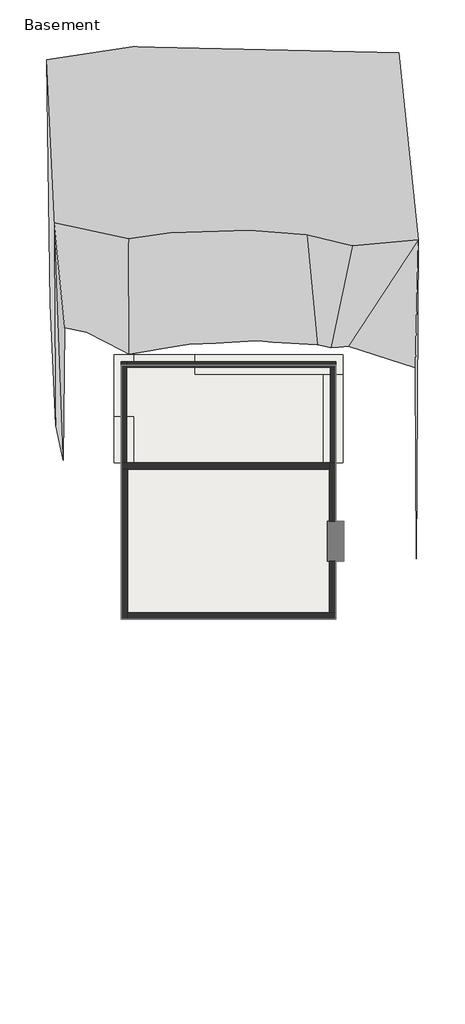
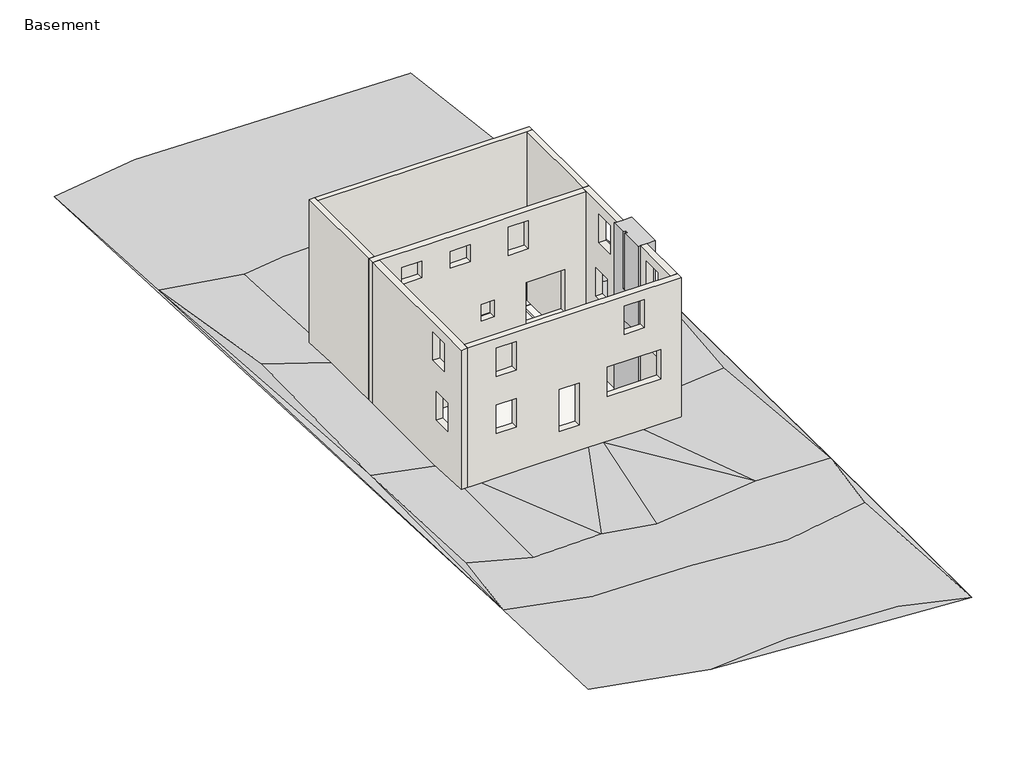
# One storey: 8 walls, 4 proxies, 3 footings, 2 slabs.
"""IFC4 building model written with IfcOpenShell, lengths in millimetres."""

import ifcopenshell
import ifcopenshell.guid

model = None  # the IFC model being written
_history = None  # IfcOwnerHistory: only IFC2X3 demands one
_inside = {}  # id of a spatial element -> (the spatial element, [elements in it])
_under = {}  # id of a project, library or spatial element -> (it, [spatial elements below it])
_declared = {}  # id of a project -> (the project, [libraries it declares])
_typed = {}  # id of a type object -> (the type object, [elements of that type])
_made_of = {}  # id of a material, layer set ... -> (it, [elements and type objects made of it])


def new_model(schema):
    """Start an empty IFC model of exactly this schema.

    Asked for "IFC4X3", IfcOpenShell would pick the latest addendum, in which some entities
    have other attributes; the version numbers below select the first issue.
    IFC2X3 requires an IfcOwnerHistory on every rooted entity: one is made here for all.
    """
    global model, _history
    if schema == "IFC4X3":
        model = ifcopenshell.file(schema_version=(4, 3, 0, 0))
    else:
        model = ifcopenshell.file(schema=schema)
    _inside.clear()
    _under.clear()
    _declared.clear()
    _typed.clear()
    _made_of.clear()
    _history = None
    if model.schema == "IFC2X3":
        org = make("IfcOrganization", Name="unknown")
        user = make(
            "IfcPersonAndOrganization",
            ThePerson=make("IfcPerson", FamilyName="unknown"),
            TheOrganization=org,
        )
        app = make(
            "IfcApplication",
            ApplicationDeveloper=org,
            Version="unknown",
            ApplicationFullName="unknown",
            ApplicationIdentifier="unknown",
        )
        _history = make(
            "IfcOwnerHistory",
            OwningUser=user,
            OwningApplication=app,
            ChangeAction="ADDED",
            CreationDate=0,
        )
    return model


def make(cls, **values):
    """One entity of the class cls with the attributes given. An attribute that is None is left unset."""
    return model.create_entity(
        cls, **{name: value for name, value in values.items() if value is not None}
    )


def rooted(cls, **values):
    """An entity with a GlobalId (a new one), such as an element, a storey or a relation."""
    return make(cls, GlobalId=ifcopenshell.guid.new(), OwnerHistory=_history, **values)


def si_unit(unit_type, name, prefix=None):
    """IfcSIUnit, for example si_unit("LENGTHUNIT", "METRE", prefix="MILLI")."""
    return make("IfcSIUnit", UnitType=unit_type, Prefix=prefix, Name=name)


def assignment(units):
    """IfcUnitAssignment: the units of a project."""
    return None if units is None else make("IfcUnitAssignment", Units=units)


def point(xyz):
    """IfcCartesianPoint."""
    return None if xyz is None else make("IfcCartesianPoint", Coordinates=xyz)


def direction(xyz):
    """IfcDirection."""
    return None if xyz is None else make("IfcDirection", DirectionRatios=xyz)


def frame(location, z_axis=None, x_axis=None):
    """IfcAxis2Placement3D, a coordinate frame: its origin and axes. An axis left out is left unset."""
    return make(
        "IfcAxis2Placement3D",
        Location=point(location),
        Axis=direction(z_axis),
        RefDirection=direction(x_axis),
    )


def origin():
    """The frame at (0, 0, 0) with its axes left unset."""
    return frame((0.0, 0.0, 0.0))


def place(relative_to, where):
    """IfcLocalPlacement: puts the frame where relative to a parent placement (None: the world)."""
    return make(
        "IfcLocalPlacement", PlacementRelTo=relative_to, RelativePlacement=where
    )


def context(
    kind, dimensions, precision=None, world=None, true_north=None, identifier=None
):
    """IfcGeometricRepresentationContext, for example the 3D "Model" context."""
    return make(
        "IfcGeometricRepresentationContext",
        ContextIdentifier=identifier,
        ContextType=kind,
        CoordinateSpaceDimension=dimensions,
        Precision=precision,
        WorldCoordinateSystem=world,
        TrueNorth=true_north,
    )


def project(units=None, contexts=None):
    """IfcProject with its units and contexts."""
    return rooted(
        "IfcProject",
        Name="project",
        RepresentationContexts=contexts,
        UnitsInContext=assignment(units),
    )


def spatial(cls, under=None, at=None, **own):
    """A site, building, storey or space (cls), placed at a placement, below another one or the project."""
    s = rooted(cls, ObjectPlacement=at, **own)
    if under is not None:
        _under.setdefault(under.id(), (under, []))[1].append(s)
    return s


def polyline(points):
    """IfcPolyline through the points."""
    return make("IfcPolyline", Points=[point(p) for p in points])


def point_list(points):
    """IfcCartesianPointList2D or 3D."""
    cls = (
        "IfcCartesianPointList2D" if len(points[0]) == 2 else "IfcCartesianPointList3D"
    )
    return make(cls, CoordList=points)


def outline(outer, holes=None, kind="AREA"):
    """IfcArbitraryClosedProfileDef: a profile drawn as a closed curve; with holes, ...WithVoids."""
    if holes is None:
        return make("IfcArbitraryClosedProfileDef", ProfileType=kind, OuterCurve=outer)
    return make(
        "IfcArbitraryProfileDefWithVoids",
        ProfileType=kind,
        OuterCurve=outer,
        InnerCurves=holes,
    )


def extrude(swept, where, along, depth):
    """IfcExtrudedAreaSolid: the profile swept, set in the frame where, extruded along a direction by depth."""
    return make(
        "IfcExtrudedAreaSolid",
        SweptArea=swept,
        Position=where,
        ExtrudedDirection=direction(along),
        Depth=depth,
    )


def faces_of(points, faces, orient=None, outer=None):
    """IfcFace entities. A face is a list of loops; a loop is a list of indices into points, from 0.

    orient and outer hold one flag for each loop. By default every Orientation is true, the
    first loop of a face is its IfcFaceOuterBound and the others are IfcFaceBound.
    """
    made = []
    for i, loops in enumerate(faces):
        bounds = []
        for j, loop in enumerate(loops):
            is_outer = j == 0 if outer is None else outer[i][j]
            bounds.append(
                make(
                    "IfcFaceOuterBound" if is_outer else "IfcFaceBound",
                    Bound=make("IfcPolyLoop", Polygon=[points[k] for k in loop]),
                    Orientation=True if orient is None else orient[i][j],
                )
            )
        made.append(make("IfcFace", Bounds=bounds))
    return made


def faceted_brep(points, faces, orient=None, outer=None, voids=None):
    """IfcFacetedBrep: a solid bounded by flat faces; with voids (closed shells), ...WithVoids."""
    shared = [point(p) for p in points]
    hull = make("IfcClosedShell", CfsFaces=faces_of(shared, faces, orient, outer))
    if voids is None:
        return make("IfcFacetedBrep", Outer=hull)
    return make(
        "IfcFacetedBrepWithVoids",
        Outer=hull,
        Voids=[
            make(cls, CfsFaces=faces_of(shared, fs, o, b)) for cls, fs, o, b in voids
        ],
    )


def triangles(points, corners, closed=None, point_numbers=None):
    """IfcTriangulatedFaceSet: each triangle names its three corners, points numbered from 1."""
    return make(
        "IfcTriangulatedFaceSet",
        Coordinates=point_list(points),
        Closed=closed,
        CoordIndex=corners,
        PnIndex=point_numbers,
    )


def shape(context_of_items, identifier, shape_type, items):
    """IfcShapeRepresentation: the items that make up one representation, for example the "Body"."""
    return make(
        "IfcShapeRepresentation",
        ContextOfItems=context_of_items,
        RepresentationIdentifier=identifier,
        RepresentationType=shape_type,
        Items=items,
    )


def source(mapping_origin, context_of_items, identifier, shape_type, items):
    """IfcRepresentationMap: a shape defined once, which mapped items show again and again."""
    return make(
        "IfcRepresentationMap",
        MappingOrigin=mapping_origin,
        MappedRepresentation=shape(context_of_items, identifier, shape_type, items),
    )


def transform(
    local_origin,
    x_axis=None,
    y_axis=None,
    z_axis=None,
    scale=None,
    scale2=None,
    scale3=None,
    uniform=True,
):
    """IfcCartesianTransformationOperator3D, or its non-uniform kind. x_axis, y_axis, z_axis: its Axis1, 2, 3."""
    if uniform:
        return make(
            "IfcCartesianTransformationOperator3D",
            Axis1=direction(x_axis),
            Axis2=direction(y_axis),
            LocalOrigin=point(local_origin),
            Scale=scale,
            Axis3=direction(z_axis),
        )
    return make(
        "IfcCartesianTransformationOperator3DnonUniform",
        Axis1=direction(x_axis),
        Axis2=direction(y_axis),
        LocalOrigin=point(local_origin),
        Scale=scale,
        Axis3=direction(z_axis),
        Scale2=scale2,
        Scale3=scale3,
    )


def mapped(mapping_source, mapping_target):
    """IfcMappedItem: shows the shape of a source again, moved by a transform."""
    return make(
        "IfcMappedItem", MappingSource=mapping_source, MappingTarget=mapping_target
    )


def made_of(thing, what):
    """Note that an element or type object is made of a material, layer set ...; save() writes the relation."""
    if what is not None:
        _made_of.setdefault(what.id(), (what, []))[1].append(thing)
    return thing


def element(
    cls,
    number,
    at=None,
    inside=None,
    cuts=None,
    type_object=None,
    material=None,
    context=None,
    identifier="Body",
    shape_type=None,
    held_by="IfcProductDefinitionShape",
    body=None,
    shapes=None,
    **own,
):
    """One element of the class cls, such as IfcWall. Its Tag is "e" and its number.

    at: its placement. inside: the storey or other place that contains it. cuts: it is an
    opening in that element (IfcRelVoidsElement). A single representation is given by context,
    identifier, shape_type and body (its items); several are given by shapes. held_by: the class
    of the entity that holds the representations. save() writes the other relations.
    """
    e = rooted(cls, Tag="e%d" % number, ObjectPlacement=at, **own)
    if body is not None:
        shapes = [shape(context, identifier, shape_type, body)]
    if shapes is not None:
        e.Representation = make(held_by, Representations=shapes)
    if inside is not None:
        _inside.setdefault(inside.id(), (inside, []))[1].append(e)
    if cuts is not None:
        rooted(
            "IfcRelVoidsElement", RelatingBuildingElement=cuts, RelatedOpeningElement=e
        )
    if type_object is not None:
        _typed.setdefault(type_object.id(), (type_object, []))[1].append(e)
    return made_of(e, material)


def aggregate(whole, parts):
    """IfcRelAggregates: a whole, such as a stair, and the parts it consists of."""
    return rooted("IfcRelAggregates", RelatingObject=whole, RelatedObjects=parts)


def save(model, path):
    """Write the relations noted so far, then the file.

    IfcRelAggregates (storeys below a building ...), IfcRelContainedInSpatialStructure (elements
    in a storey), IfcRelDefinesByType, IfcRelAssociatesMaterial and IfcRelDeclares: one each for
    every whole, place, type object, material and project.
    """
    for whole, parts in _under.values():
        aggregate(whole, parts)
    for where, things in _inside.values():
        rooted(
            "IfcRelContainedInSpatialStructure",
            RelatedElements=things,
            RelatingStructure=where,
        )
    for kind, things in _typed.values():
        rooted("IfcRelDefinesByType", RelatedObjects=things, RelatingType=kind)
    for what, things in _made_of.values():
        rooted("IfcRelAssociatesMaterial", RelatedObjects=things, RelatingMaterial=what)
    for by, libraries in _declared.values():
        rooted("IfcRelDeclares", RelatingContext=by, RelatedDefinitions=libraries)
    model.write(path)


def existing_fireplace_existing_fireplace_063a625f(model_context):
    return source(origin(), model_context, "Body", "Brep", [
        faceted_brep([(4450.2196932, 434.2888758, 5486.4), (4069.2196932, 434.2888758, 5486.4), (3764.4196932, 434.2888758, 5486.4), (3662.8196932, 434.2888758, 5486.4), (3662.8196932, -276.9111242, 5486.4), (3767.2567114, -276.9111242, 5486.4), (3767.2567114, -403.9111242, 5486.4), (3662.8196932, -403.9111242, 5486.4), (3662.8196932, -1445.3111242, 5486.4), (3764.4196932, -1445.3111242, 5486.4), (4069.2196932, -1445.3111242, 5486.4), (4450.2196932, -1445.3111242, 5486.4), (4450.2196932, 434.2888758, -2667.0), (4450.2196932, -1445.3111242, -2667.0), (4069.2196932, -1445.3111242, -2667.0), (3764.4196932, -1445.3111242, -2667.0), (3662.8196932, -1445.3111242, -2667.0), (3662.8196932, 434.2888758, -2667.0), (3764.4196932, 434.2888758, -2667.0), (4069.2196932, 434.2888758, -2667.0), (3662.8196932, -403.9111242, 2743.2), (3662.8196932, -276.9111242, 2743.2), (3662.8196932, 154.8888758, 0.0), (3662.8196932, 154.8888758, 1219.2), (3662.8196932, -1165.9111242, 1219.2), (3662.8196932, -1165.9111242, 0.0), (4145.4196932, -20.7631592, 1219.2), (4145.4196932, -990.2590891, 1219.2), (4145.4196932, -990.2590891, 0.0), (4145.4196932, -20.7631592, 0.0), (3767.2567114, -403.9111242, 2743.2), (3767.2567114, -276.9111242, 2743.2)], [[[0, 1, 2, 3, 4, 5, 6, 7, 8, 9, 10, 11]], [[12, 13, 14, 15, 16, 17, 18, 19]], [[3, 2, 1, 0, 12, 19, 18, 17]], [[3, 17, 16, 8, 7, 20, 21, 4], [22, 23, 24, 25]], [[11, 10, 9, 8, 16, 15, 14, 13]], [[0, 11, 13, 12]], [[24, 23, 26, 27]], [[25, 24, 27, 28]], [[27, 26, 29, 28]], [[23, 22, 29, 26]], [[22, 25, 28, 29]], [[6, 30, 20, 7]], [[31, 5, 4, 21]], [[30, 31, 21, 20]], [[30, 6, 5, 31]]]),
    ])


model = new_model("IFC4")

# Units and contexts
model_context = context("Model", 3, world=origin())
ifc_project = project(units=[si_unit("LENGTHUNIT", "METRE", prefix="MILLI")], contexts=[model_context])

# Site, building, storey
site = spatial("IfcSite", under=ifc_project)
building = spatial("IfcBuilding", under=site)
storey = spatial("IfcBuildingStorey", under=building, Name="Basement", Elevation=-2667.0)

# Proxies
placement = place(None, origin())
element("IfcBuildingElementProxy", 1, Name="Building Element Proxy", at=placement, inside=storey, context=model_context, shape_type="Tessellation", body=[
    triangles([(-9474.14729, 22003.2871765, -1727.1999516), (-8916.1412338, -12566.1132111, -939.7999758), (-8632.7724838, -18803.3999359, -1092.1999758), (-3754.3850807, -20036.8885986, -1092.1999758), (7677.2023224, -20906.8378235, -1092.1999758), (7936.7585724, 13587.9496765, -1752.6), (7012.0400162, 22339.8364014, -1727.1999516), (-5437.1349838, 22620.8239014, -1727.1999516), (4069.2196426, 434.2888621, -1346.1999516), (4450.2196426, 434.2888621, -1346.1999516), (4450.2196426, -349.5066825, -1346.1999516), (4450.2196426, -1445.3110531, -1346.1999516), (4069.2196426, -1445.3110531, -1346.1999516), (4069.2196426, -2313.9084709, -1346.1999516), (4069.2196426, -4163.1110046, -1246.6980309), (3428.5651428, -4163.1110046, -1250.4688763), (2349.5500454, -4163.1110046, -1257.7835461), (502.5996998, -4163.1110046, -1235.211668), (-175.7374563, -4163.1110046, -1228.3558365), (-2922.786422, -4163.1110046, -1226.4072636), (-5055.1879486, -4163.1110046, -1242.8984081), (-5852.784613, -4163.1110046, -1243.6517052), (-5989.1803574, -4163.1110046, -1240.8027512), (-5989.1803574, -2711.9263275, -1314.8636375), (-5989.1803574, -2124.4043404, -1346.1999516), (-5989.1803574, 3152.0889954, -1346.1999516), (-5989.1803574, 4989.0600082, -1346.1999516), (-5989.1803574, 6156.3282944, -1346.1999516), (-5989.1803574, 7724.0889954, -1429.2445919), (-5611.7969971, 7724.0889954, -1439.6358181), (-2815.8938187, 7724.0889954, -1415.0254017), (-2474.4123367, 7724.0889954, -1412.4145145), (-1876.9665367, 7724.0889954, -1411.4359406), (391.3462071, 7724.0889954, -1403.6252254), (781.867392, 7724.0889954, -1405.4288944), (3306.7437996, 7724.0889954, -1413.4377079), (3676.8014442, 7724.0889954, -1418.4369667), (4069.2196426, 7724.0889954, -1416.2554138), (4069.2196426, 7529.9159637, -1404.4058464), (4069.2196426, 6299.0253983, -1346.1999516), (4069.2196426, 3152.0889954, -1346.1999516), (-9109.81604, 14372.1750641, -1752.6), (-8549.4287338, -9013.2876297, -939.7999758), (-8523.2349838, -1401.2252266, -1346.1999516), (-8408.9349838, 7414.1625641, -1346.1999516), (-6082.4537338, -10022.9382111, -939.7999758), (-5633.19104, 13643.5125641, -1752.6), (-5382.3662338, -13518.6132111, -939.7999758), (-3671.0413307, 13924.5000641, -1752.6), (-2942.3788307, -9965.7882111, -939.7999758), (-1568.3975807, 21947.7254517, -1727.1999516), (-840.5287823, -13629.7378235, -939.7999758), (-699.241258, -10470.6132111, -939.7999758), (-109.4850414, -19700.3370483, -1092.1999758), (29.4212079, 14035.6246765, -1752.6), (2721.8210724, 13811.7871765, -1752.6), (2805.1648224, 21892.1614014, -1727.1999516), (3252.0462662, -14021.8499359, -939.7999758), (4179.1460724, -9854.6624359, -939.7999758), (4845.1025162, -19962.2745483, -1092.1999758), (4852.2462662, 13306.9621765, -1752.6), (7177.93396, -13294.7757111, -939.7999758), (7289.85271, -1961.6126781, -1346.1999516), (7543.0587662, -9965.7882111, -939.7999758), (7740.7025162, 5059.8998703, -1346.1999516)], [[46, 2, 48], [43, 46, 23], [46, 43, 2], [2, 3, 48], [2, 43, 44], [43, 23, 44], [23, 46, 22], [44, 23, 24], [46, 21, 22], [44, 24, 25], [48, 4, 52], [4, 48, 3], [48, 52, 50], [19, 53, 18], [4, 54, 52], [50, 52, 53], [21, 50, 20], [21, 46, 50], [19, 20, 50], [50, 53, 19], [53, 52, 58], [50, 46, 48], [45, 27, 28], [26, 27, 45], [44, 26, 45], [25, 26, 44], [8, 1, 42], [1, 2, 42], [42, 45, 47], [29, 45, 28], [42, 44, 45], [29, 47, 45], [42, 2, 44], [47, 30, 31], [31, 32, 49], [33, 49, 32], [47, 8, 42], [8, 47, 49], [49, 51, 8], [55, 51, 49], [47, 31, 49], [8, 51, 57], [55, 49, 33], [30, 47, 29], [58, 59, 53], [58, 54, 60], [59, 15, 16], [59, 18, 53], [16, 17, 59], [59, 17, 18], [12, 13, 14], [14, 15, 63], [58, 62, 59], [62, 60, 5], [64, 5, 65], [5, 64, 62], [60, 54, 5], [59, 62, 64], [59, 64, 15], [12, 63, 11], [12, 14, 63], [64, 63, 15], [11, 63, 10], [64, 65, 63], [62, 58, 60], [54, 4, 5], [55, 34, 35], [56, 35, 36], [55, 56, 57], [55, 35, 56], [37, 61, 36], [56, 61, 57], [56, 36, 61], [55, 57, 51], [55, 33, 34], [40, 41, 65], [10, 65, 41], [65, 10, 63], [41, 9, 10], [40, 65, 39], [39, 65, 38], [61, 6, 7], [6, 61, 38], [61, 7, 57], [65, 6, 38], [38, 61, 37], [65, 5, 6], [57, 7, 8], [52, 54, 58]], closed=False),
])
element("IfcBuildingElementProxy", 2, Name="Building Element Proxy", at=placement, inside=storey, context=model_context, shape_type="Tessellation", body=[
    triangles([(4069.2196426, 3152.0889954, -3073.5594864), (4069.2196426, 3152.0889954, -1346.1999516), (4069.2196426, 434.2888621, -3073.5594864), (4069.2196426, 434.2888621, -1346.1999516), (4450.2196426, 434.2888621, -3073.5594864), (4450.2196426, 434.2888621, -1346.1999516), (4450.2196426, -349.5066825, -3073.5594864), (4450.2196426, -349.5066825, -1346.1999516), (4450.2196426, -1445.3110531, -3073.5594864), (4450.2196426, -1445.3110531, -1346.1999516), (4069.2196426, -1445.3110531, -3073.5594864), (4069.2196426, -1445.3110531, -1346.1999516), (4069.2196426, -2313.9084709, -3073.5594864), (4069.2196426, -2313.9084709, -1346.1999516), (4069.2196426, -4163.1110046, -3073.5594864), (4069.2196426, -4163.1110046, -1246.6980309), (3428.5651428, -4163.1110046, -3073.5594864), (3428.5651428, -4163.1110046, -1250.4688763), (2349.5500454, -4163.1110046, -3073.5594864), (2349.5500454, -4163.1110046, -1257.7835461), (502.5996998, -4163.1110046, -3073.5594864), (502.5996998, -4163.1110046, -1235.211668), (-175.7374563, -4163.1110046, -3073.5594864), (-175.7374563, -4163.1110046, -1228.3558365), (-2922.786422, -4163.1110046, -3073.5594864), (-2922.786422, -4163.1110046, -1226.4072636), (-5055.1879486, -4163.1110046, -3073.5594864), (-5055.1879486, -4163.1110046, -1242.8984081), (-5852.784613, -4163.1110046, -3073.5594864), (-5852.784613, -4163.1110046, -1243.6517052), (-5989.1803574, -4163.1110046, -3073.5594864), (-5989.1803574, -4163.1110046, -1240.8027512), (-5989.1803574, -2711.9263275, -3073.5594864), (-5989.1803574, -2711.9263275, -1314.8636375), (-5989.1803574, -2124.4043404, -3073.5594864), (-5989.1803574, -2124.4043404, -1346.1999516), (-5989.1803574, 3152.0889954, -3073.5594864), (-5989.1803574, 3152.0889954, -1346.1999516)], [[1, 4, 2], [1, 3, 4], [3, 6, 4], [3, 5, 6], [5, 8, 6], [5, 7, 8], [7, 10, 8], [7, 9, 10], [9, 12, 10], [9, 11, 12], [11, 14, 12], [11, 13, 14], [13, 16, 14], [13, 15, 16], [15, 18, 16], [15, 17, 18], [17, 20, 18], [17, 19, 20], [19, 22, 20], [19, 21, 22], [21, 24, 22], [21, 23, 24], [23, 26, 24], [23, 25, 26], [25, 28, 26], [25, 27, 28], [27, 30, 28], [27, 29, 30], [29, 32, 30], [29, 31, 32], [31, 34, 32], [31, 33, 34], [33, 36, 34], [33, 35, 36], [35, 38, 36], [35, 37, 38]], closed=False),
    triangles([(4069.2196426, 434.2888621, -3073.5594864), (4069.2196426, 3152.0889954, -3073.5594864), (-5989.1803574, 3152.0889954, -3073.5594864), (-5989.1803574, -4163.1110046, -3073.5594864), (4069.2196426, -4163.1110046, -3073.5594864), (4069.2196426, -1445.3110531, -3073.5594864), (4450.2196426, -1445.3110531, -3073.5594864), (4450.2196426, 434.2888621, -3073.5594864)], [[4, 6, 3], [6, 4, 5], [3, 1, 2], [1, 3, 6], [6, 7, 1], [8, 1, 7]], closed=False),
])
element("IfcBuildingElementProxy", 3, Name="Building Element Proxy", at=placement, inside=storey, context=model_context, shape_type="Tessellation", body=[
    triangles([(-5989.1803574, 3152.0889954, -3073.5594864), (-5989.1803574, 3152.0889954, -1346.1999516), (-5989.1803574, 4989.0600082, -3073.5594864), (-5989.1803574, 4989.0600082, -1346.1999516), (-5989.1803574, 6156.3282944, -3073.5594864), (-5989.1803574, 6156.3282944, -1346.1999516), (-5989.1803574, 7724.0889954, -3073.5594864), (-5989.1803574, 7724.0889954, -1429.2445919), (-5611.7969971, 7724.0889954, -3073.5594864), (-5611.7969971, 7724.0889954, -1439.6358181), (-2815.8938187, 7724.0889954, -3073.5594864), (-2815.8938187, 7724.0889954, -1415.0254017), (-2474.4123367, 7724.0889954, -3073.5594864), (-2474.4123367, 7724.0889954, -1412.4145145), (-1876.9665367, 7724.0889954, -3073.5594864), (-1876.9665367, 7724.0889954, -1411.4359406), (391.3462071, 7724.0889954, -3073.5594864), (391.3462071, 7724.0889954, -1403.6252254), (781.867392, 7724.0889954, -3073.5594864), (781.867392, 7724.0889954, -1405.4288944), (3306.7437996, 7724.0889954, -3073.5594864), (3306.7437996, 7724.0889954, -1413.4377079), (3676.8014442, 7724.0889954, -3073.5594864), (3676.8014442, 7724.0889954, -1418.4369667), (4069.2196426, 7724.0889954, -3073.5594864), (4069.2196426, 7724.0889954, -1416.2554138), (4069.2196426, 7529.9159637, -3073.5594864), (4069.2196426, 7529.9159637, -1404.4058464), (4069.2196426, 6299.0253983, -3073.5594864), (4069.2196426, 6299.0253983, -1346.1999516), (4069.2196426, 3152.0889954, -3073.5594864), (4069.2196426, 3152.0889954, -1346.1999516)], [[1, 4, 2], [1, 3, 4], [3, 6, 4], [3, 5, 6], [5, 8, 6], [5, 7, 8], [7, 10, 8], [7, 9, 10], [9, 12, 10], [9, 11, 12], [11, 14, 12], [11, 13, 14], [13, 16, 14], [13, 15, 16], [15, 18, 16], [15, 17, 18], [17, 20, 18], [17, 19, 20], [19, 22, 20], [19, 21, 22], [21, 24, 22], [21, 23, 24], [23, 26, 24], [23, 25, 26], [25, 28, 26], [25, 27, 28], [27, 30, 28], [27, 29, 30], [29, 32, 30], [29, 31, 32]], closed=False),
    triangles([(-5989.1803574, 7724.0889954, -3073.5594864), (-5989.1803574, 3152.0889954, -3073.5594864), (4069.2196426, 3152.0889954, -3073.5594864), (4069.2196426, 7724.0889954, -3073.5594864)], [[1, 2, 4], [3, 4, 2]], closed=False),
])
existing_fireplace_existing_fireplace_shape = existing_fireplace_existing_fireplace_063a625f(model_context)
element("IfcBuildingElementProxy", 4, Name="Existing Fireplace : Existing Fireplace", ObjectType="Existing Fireplace : Existing Fireplace", at=placement, inside=storey, context=model_context, shape_type="MappedRepresentation", body=[
    mapped(existing_fireplace_existing_fireplace_shape, transform((0.0, 0.0, 0.0), x_axis=(1.0, 0.0, 0.0), y_axis=(0.0, 1.0, 0.0), z_axis=(0.0, 0.0, 1.0))),
])

# Footings
element("IfcFooting", 5, ObjectType="Bearing Footing - 36\" x 12\"", at=placement, inside=storey, context=model_context, shape_type="Brep", body=[
    faceted_brep([(-5404.9803068, 3152.0888758, -2667.0), (-6319.3803068, 3152.0888758, -2667.0), (-6319.3803068, 3152.0888758, -2971.8), (-5404.9803068, 3152.0888758, -2971.8), (-6319.3803068, 5311.0888758, -2667.0), (-5404.9803068, 5311.0888758, -2667.0), (-5404.9803068, 5311.0888758, -2971.8), (-6319.3803068, 5311.0888758, -2971.8)], [[[0, 1, 2, 3]], [[4, 5, 6, 7]], [[0, 5, 4, 1]], [[2, 1, 4, 7]], [[3, 2, 7, 6]], [[0, 3, 6, 5]]]),
    faceted_brep([(-5404.9803068, 5311.0888758, -3124.2), (-6319.3803068, 5311.0888758, -3124.2), (-6319.3803068, 5311.0888758, -3429.0), (-5404.9803068, 5311.0888758, -3429.0), (-5404.9803068, 7292.2888758, -3124.2), (-5404.9803068, 8206.6888758, -3124.2), (-6319.3803068, 8206.6888758, -3124.2), (-6319.3803068, 8206.6888758, -3429.0), (-5404.9803068, 8206.6888758, -3429.0), (-5404.9803068, 7292.2888758, -3429.0)], [[[0, 1, 2, 3]], [[0, 4, 5, 6, 1]], [[2, 1, 6, 7]], [[3, 2, 7, 8, 9]], [[0, 3, 9, 8, 5, 4]], [[6, 5, 8, 7]]]),
])
element("IfcFooting", 6, ObjectType="Bearing Footing - 36\" x 12\"", at=placement, inside=storey, context=model_context, shape_type="Brep", body=[
    faceted_brep([(-2509.3803068, 8206.6888758, -3429.0), (-2509.3803068, 8206.6888758, -3124.2), (-2509.3803068, 7292.2888758, -3124.2), (-2509.3803068, 7292.2888758, -3429.0), (-5404.9803068, 8206.6888758, -3124.2), (-5404.9803068, 7292.2888758, -3124.2), (-5404.9803068, 8206.6888758, -3429.0), (-5404.9803068, 7292.2888758, -3429.0)], [[[0, 1, 2, 3]], [[2, 1, 4, 5]], [[1, 0, 6, 4]], [[0, 3, 7, 6]], [[3, 2, 5, 7]], [[5, 4, 6, 7]]]),
    faceted_brep([(-2509.3803068, 8206.6888758, -2667.0), (-2509.3803068, 8206.6888758, -2971.8), (-2509.3803068, 7292.2888758, -2971.8), (-2509.3803068, 7292.2888758, -2667.0), (4399.4196932, 8206.6888758, -2667.0), (3485.0196932, 7292.2888758, -2667.0), (4399.4196932, 7292.2888758, -2667.0), (4399.4196932, 8206.6888758, -2971.8), (4399.4196932, 7292.2888758, -2971.8), (3485.0196932, 7292.2888758, -2971.8)], [[[0, 1, 2, 3]], [[4, 0, 3, 5, 6]], [[1, 0, 4, 7]], [[2, 1, 7, 8, 9]], [[3, 2, 9, 8, 6, 5]], [[4, 6, 8, 7]]]),
])
element("IfcFooting", 7, ObjectType="Bearing Footing - 36\" x 12\"", at=placement, inside=storey, context=model_context, shape_type="SweptSolid", body=[
    extrude(outline(polyline([(4399.4196932, 3152.0888758), (3485.0196932, 3152.0888758), (3485.0196932, 7292.2888758), (4399.4196932, 7292.2888758), (4399.4196932, 3152.0888758)])), frame((0.0, 0.0, -2971.8), z_axis=(0.0, 0.0, 1.0), x_axis=(1.0, 0.0, 0.0)), (0.0, 0.0, 1.0), 304.8),
])

# Slabs
element("IfcSlab", 8, ObjectType="Pad 1", at=placement, inside=storey, context=model_context, shape_type="SweptSolid", body=[
    extrude(outline(polyline([(4069.2196932, 434.2888758), (4450.2196932, 434.2888758), (4450.2196932, -1445.3111242), (4069.2196932, -1445.3111242), (4069.2196932, -4163.1111242), (-5989.1803068, -4163.1111242), (-5989.1803068, 3152.0888758), (4069.2196932, 3152.0888758), (4069.2196932, 434.2888758)])), frame((0.0, 0.0, -3073.4), z_axis=(0.0, 0.0, 1.0), x_axis=(1.0, 0.0, 0.0)), (0.0, 0.0, 1.0), 304.8),
])
element("IfcSlab", 9, ObjectType="Pad 1", at=placement, inside=storey, context=model_context, shape_type="SweptSolid", body=[
    extrude(outline(polyline([(-5989.1803068, 7724.0888758), (4069.2196932, 7724.0888758), (4069.2196932, 3152.0888758), (-5989.1803068, 3152.0888758), (-5989.1803068, 7724.0888758)])), frame((0.0, 0.0, -3073.4), z_axis=(0.0, 0.0, 1.0), x_axis=(1.0, 0.0, 0.0)), (0.0, 0.0, 1.0), 304.8),
])

# Walls
element("IfcWall", 10, ObjectType="Generic - 10\"", at=placement, inside=storey, context=model_context, shape_type="Brep", body=[
    faceted_brep([(-5735.1803068, 3152.0888758, -2667.0), (-5735.1803068, 5311.0888758, -2667.0), (-5735.1803068, 5311.0888758, -3124.2), (-5735.1803068, 7622.4888758, -3124.2), (-5735.1803068, 7876.4888758, -3124.2), (-5735.1803068, 7876.4888758, 5486.4), (-5735.1803068, 7622.4888758, 5486.4), (-5735.1803068, 3152.0888758, 5486.4), (-5989.1803068, 3152.0888758, -2667.0), (-5989.1803068, 3152.0888758, 5486.4), (-5989.1803068, 7876.4888758, 5486.4), (-5989.1803068, 7876.4888758, -3124.2), (-5989.1803068, 5311.0888758, -3124.2), (-5989.1803068, 5311.0888758, -2667.0)], [[[0, 1, 2, 3, 4, 5, 6, 7]], [[8, 9, 10, 11, 12, 13]], [[1, 0, 8, 13]], [[2, 1, 13, 12]], [[4, 3, 2, 12, 11]], [[7, 6, 5, 10, 9]], [[5, 4, 11, 10]], [[0, 7, 9, 8]]]),
])
element("IfcWall", 11, ObjectType="Generic - 10\"", at=placement, inside=storey, context=model_context, shape_type="Brep", body=[
    faceted_brep([(-5735.1803068, 7622.4888758, -3124.2), (-2509.3803068, 7622.4888758, -3124.2), (-2509.3803068, 7622.4888758, -2667.0), (3815.2196932, 7622.4888758, -2667.0), (4069.2196932, 7622.4888758, -2667.0), (4069.2196932, 7622.4888758, 5486.4), (3815.2196932, 7622.4888758, 5486.4), (-5735.1803068, 7622.4888758, 5486.4), (-5735.1803068, 7876.4888758, -3124.2), (-5735.1803068, 7876.4888758, 5486.4), (4069.2196932, 7876.4888758, 5486.4), (4069.2196932, 7876.4888758, -2667.0), (-2509.3803068, 7876.4888758, -2667.0), (-2509.3803068, 7876.4888758, -3124.2)], [[[0, 1, 2, 3, 4, 5, 6, 7]], [[8, 9, 10, 11, 12, 13]], [[1, 0, 8, 13]], [[2, 1, 13, 12]], [[4, 3, 2, 12, 11]], [[7, 6, 5, 10, 9]], [[5, 4, 11, 10]], [[0, 7, 9, 8]]]),
])
element("IfcWall", 12, ObjectType="Generic - 10\"", at=placement, inside=storey, context=model_context, shape_type="SweptSolid", body=[
    extrude(outline(polyline([(3815.2196932, 3152.0888758), (3815.2196932, 7622.4888758), (4069.2196932, 7622.4888758), (4069.2196932, 3152.0888758), (3815.2196932, 3152.0888758)])), frame((0.0, 0.0, -2667.0), z_axis=(0.0, 0.0, 1.0), x_axis=(1.0, 0.0, 0.0)), (0.0, 0.0, 1.0), 8153.4),
])
element("IfcWall", 13, ObjectType="Generic - 12\"", at=placement, inside=storey, context=model_context, shape_type="Brep", body=[
    faceted_brep([(-5989.1803068, 2847.2888758, -2667.0), (-5684.3803068, 2847.2888758, -2667.0), (3764.4196932, 2847.2888758, -2667.0), (3764.4196932, 2847.2888758, 5486.4), (56.0196932, 2847.2888758, 5486.4), (-70.9803068, 2847.2888758, 5486.4), (-680.5803068, 2847.2888758, 5486.4), (-807.5803068, 2847.2888758, 5486.4), (-3169.7803068, 2847.2888758, 5486.4), (-3296.7803068, 2847.2888758, 5486.4), (-5684.3803068, 2847.2888758, 5486.4), (-5989.1803068, 2847.2888758, 5486.4), (1021.2196932, 2847.2888758, 0.0), (1021.2196932, 2847.2888758, 2057.4), (2799.2196932, 2847.2888758, 2057.4), (2799.2196932, 2847.2888758, 0.0), (-4160.3803068, 2847.2888758, 0.0), (-5023.9803068, 2847.2888758, 0.0), (-5023.9803068, 2847.2888758, 2032.0), (-4160.3803068, 2847.2888758, 2032.0), (-1036.1803068, 2847.2888758, 914.4), (-1036.1803068, 2847.2888758, 1727.2), (-426.5803068, 2847.2888758, 1727.2), (-426.5803068, 2847.2888758, 914.4), (-3919.0803068, 2847.2888758, 914.4), (-3919.0803068, 2847.2888758, 1727.2), (-3004.6803068, 2847.2888758, 1727.2), (-3004.6803068, 2847.2888758, 914.4), (208.4196932, 2847.2888758, 3657.6), (208.4196932, 2847.2888758, 5029.2), (1122.8196932, 2847.2888758, 5029.2), (1122.8196932, 2847.2888758, 3657.6), (-2433.1803068, 2847.2888758, 3962.4), (-2433.1803068, 2847.2888758, 4775.2), (-1518.7803068, 2847.2888758, 4775.2), (-1518.7803068, 2847.2888758, 3962.4), (-4668.3803068, 2847.2888758, 3962.4), (-4668.3803068, 2847.2888758, 4775.2), (-3753.9803068, 2847.2888758, 4775.2), (-3753.9803068, 2847.2888758, 3962.4), (3764.4196932, 3152.0888758, -2667.0), (-5989.1803068, 3152.0888758, -2667.0), (-5989.1803068, 3152.0888758, 5486.4), (3764.4196932, 3152.0888758, 5486.4), (1021.2196932, 3152.0888758, 2057.4), (1021.2196932, 3152.0888758, 0.0), (2799.2196932, 3152.0888758, 0.0), (2799.2196932, 3152.0888758, 2057.4), (-5023.9803068, 3152.0888758, 0.0), (-4160.3803068, 3152.0888758, 0.0), (-4160.3803068, 3152.0888758, 2032.0), (-5023.9803068, 3152.0888758, 2032.0), (-1036.1803068, 3152.0888758, 1727.2), (-1036.1803068, 3152.0888758, 914.4), (-426.5803068, 3152.0888758, 914.4), (-426.5803068, 3152.0888758, 1727.2), (-3919.0803068, 3152.0888758, 1727.2), (-3919.0803068, 3152.0888758, 914.4), (-3004.6803068, 3152.0888758, 914.4), (-3004.6803068, 3152.0888758, 1727.2), (208.4196932, 3152.0888758, 5029.2), (208.4196932, 3152.0888758, 3657.6), (1122.8196932, 3152.0888758, 3657.6), (1122.8196932, 3152.0888758, 5029.2), (-2433.1803068, 3152.0888758, 4775.2), (-2433.1803068, 3152.0888758, 3962.4), (-1518.7803068, 3152.0888758, 3962.4), (-1518.7803068, 3152.0888758, 4775.2), (-4668.3803068, 3152.0888758, 4775.2), (-4668.3803068, 3152.0888758, 3962.4), (-3753.9803068, 3152.0888758, 3962.4), (-3753.9803068, 3152.0888758, 4775.2)], [[[0, 1, 2, 3, 4, 5, 6, 7, 8, 9, 10, 11], [12, 13, 14, 15], [16, 17, 18, 19], [20, 21, 22, 23], [24, 25, 26, 27], [28, 29, 30, 31], [32, 33, 34, 35], [36, 37, 38, 39]], [[40, 41, 42, 43], [44, 45, 46, 47], [48, 49, 50, 51], [52, 53, 54, 55], [56, 57, 58, 59], [60, 61, 62, 63], [64, 65, 66, 67], [68, 69, 70, 71]], [[2, 1, 0, 41, 40]], [[11, 10, 9, 8, 7, 6, 5, 4, 3, 43, 42]], [[0, 11, 42, 41]], [[3, 2, 40, 43]], [[44, 13, 12, 45]], [[13, 44, 47, 14]], [[14, 47, 46, 15]], [[45, 12, 15, 46]], [[17, 16, 49, 48]], [[18, 17, 48, 51]], [[19, 18, 51, 50]], [[16, 19, 50, 49]], [[53, 52, 21, 20]], [[54, 53, 20, 23]], [[55, 54, 23, 22]], [[52, 55, 22, 21]], [[57, 56, 25, 24]], [[58, 57, 24, 27]], [[59, 58, 27, 26]], [[56, 59, 26, 25]], [[60, 29, 28, 61]], [[61, 28, 31, 62]], [[62, 31, 30, 63]], [[29, 60, 63, 30]], [[33, 32, 65, 64]], [[32, 35, 66, 65]], [[35, 34, 67, 66]], [[34, 33, 64, 67]], [[37, 36, 69, 68]], [[36, 39, 70, 69]], [[39, 38, 71, 70]], [[38, 37, 68, 71]]]),
])
element("IfcWall", 14, ObjectType="Generic - 12\"", at=placement, inside=storey, context=model_context, shape_type="Brep", body=[
    faceted_brep([(-5684.3803068, -4163.1111242, -2667.0), (-5684.3803068, -3858.3111242, -2667.0), (-5684.3803068, 2847.2888758, -2667.0), (-5684.3803068, 2847.2888758, 5486.4), (-5684.3803068, 1450.2888758, 5486.4), (-5684.3803068, 1323.2888758, 5486.4), (-5684.3803068, -3858.3111242, 5486.4), (-5684.3803068, -4163.1111242, 5486.4), (-5684.3803068, -3096.3111242, 914.4), (-5684.3803068, -3096.3111242, 2286.0), (-5684.3803068, -2181.9111242, 2286.0), (-5684.3803068, -2181.9111242, 914.4), (-5684.3803068, -2842.3111242, 3657.6), (-5684.3803068, -2842.3111242, 5029.2), (-5684.3803068, -1927.9111242, 5029.2), (-5684.3803068, -1927.9111242, 3657.6), (-5989.1803068, 2847.2888758, -2667.0), (-5989.1803068, -4163.1111242, -2667.0), (-5989.1803068, -4163.1111242, 5486.4), (-5989.1803068, 2847.2888758, 5486.4), (-5989.1803068, -3096.3111242, 2286.0), (-5989.1803068, -3096.3111242, 914.4), (-5989.1803068, -2181.9111242, 914.4), (-5989.1803068, -2181.9111242, 2286.0), (-5989.1803068, -2842.3111242, 5029.2), (-5989.1803068, -2842.3111242, 3657.6), (-5989.1803068, -1927.9111242, 3657.6), (-5989.1803068, -1927.9111242, 5029.2)], [[[0, 1, 2, 3, 4, 5, 6, 7], [8, 9, 10, 11], [12, 13, 14, 15]], [[16, 17, 18, 19], [20, 21, 22, 23], [24, 25, 26, 27]], [[2, 1, 0, 17, 16]], [[7, 6, 5, 4, 3, 19, 18]], [[0, 7, 18, 17]], [[3, 2, 16, 19]], [[21, 20, 9, 8]], [[22, 21, 8, 11]], [[23, 22, 11, 10]], [[20, 23, 10, 9]], [[24, 13, 12, 25]], [[25, 12, 15, 26]], [[26, 15, 14, 27]], [[13, 24, 27, 14]]]),
])
element("IfcWall", 15, ObjectType="Generic - 12\"", at=placement, inside=storey, context=model_context, shape_type="Brep", body=[
    faceted_brep([(4069.2196932, -3858.3111242, -2667.0), (3764.4196932, -3858.3111242, -2667.0), (-5684.3803068, -3858.3111242, -2667.0), (-5684.3803068, -3858.3111242, 5486.4), (-2179.1803068, -3858.3111242, 5486.4), (-2052.1803068, -3858.3111242, 5486.4), (-807.5803068, -3858.3111242, 5486.4), (-680.5803068, -3858.3111242, 5486.4), (-70.9803068, -3858.3111242, 5486.4), (56.0196932, -3858.3111242, 5486.4), (3764.4196932, -3858.3111242, 5486.4), (4069.2196932, -3858.3111242, 5486.4), (-1518.7803068, -3858.3111242, 0.0), (-604.3803068, -3858.3111242, 0.0), (-604.3803068, -3858.3111242, 2032.0), (-1518.7803068, -3858.3111242, 2032.0), (-3474.5803068, -3858.3111242, 914.4), (-3474.5803068, -3858.3111242, 2286.0), (-4388.9803068, -3858.3111242, 2286.0), (-4388.9803068, -3858.3111242, 914.4), (691.0196932, -3858.3111242, 2336.8), (691.0196932, -3858.3111242, 914.4), (3129.4196932, -3858.3111242, 914.4), (3129.4196932, -3858.3111242, 2336.8), (2367.4196932, -3858.3111242, 3657.6), (2367.4196932, -3858.3111242, 5029.2), (1453.0196932, -3858.3111242, 5029.2), (1453.0196932, -3858.3111242, 3657.6), (-3474.5803068, -3858.3111242, 3657.6), (-3474.5803068, -3858.3111242, 5029.2), (-4388.9803068, -3858.3111242, 5029.2), (-4388.9803068, -3858.3111242, 3657.6), (-5684.3803068, -4163.1111242, -2667.0), (4069.2196932, -4163.1111242, -2667.0), (4069.2196932, -4163.1111242, 5486.4), (-5684.3803068, -4163.1111242, 5486.4), (-604.3803068, -4163.1111242, 0.0), (-1518.7803068, -4163.1111242, 0.0), (-1518.7803068, -4163.1111242, 2032.0), (-604.3803068, -4163.1111242, 2032.0), (-3474.5803068, -4163.1111242, 2286.0), (-3474.5803068, -4163.1111242, 914.4), (-4388.9803068, -4163.1111242, 914.4), (-4388.9803068, -4163.1111242, 2286.0), (691.0196932, -4163.1111242, 914.4), (691.0196932, -4163.1111242, 2336.8), (3129.4196932, -4163.1111242, 2336.8), (3129.4196932, -4163.1111242, 914.4), (2367.4196932, -4163.1111242, 5029.2), (2367.4196932, -4163.1111242, 3657.6), (1453.0196932, -4163.1111242, 3657.6), (1453.0196932, -4163.1111242, 5029.2), (-3474.5803068, -4163.1111242, 5029.2), (-3474.5803068, -4163.1111242, 3657.6), (-4388.9803068, -4163.1111242, 3657.6), (-4388.9803068, -4163.1111242, 5029.2)], [[[0, 1, 2, 3, 4, 5, 6, 7, 8, 9, 10, 11], [12, 13, 14, 15], [16, 17, 18, 19], [20, 21, 22, 23], [24, 25, 26, 27], [28, 29, 30, 31]], [[32, 33, 34, 35], [36, 37, 38, 39], [40, 41, 42, 43], [44, 45, 46, 47], [48, 49, 50, 51], [52, 53, 54, 55]], [[2, 1, 0, 33, 32]], [[11, 10, 9, 8, 7, 6, 5, 4, 3, 35, 34]], [[0, 11, 34, 33]], [[3, 2, 32, 35]], [[37, 36, 13, 12]], [[38, 37, 12, 15]], [[39, 38, 15, 14]], [[36, 39, 14, 13]], [[41, 40, 17, 16]], [[42, 41, 16, 19]], [[43, 42, 19, 18]], [[40, 43, 18, 17]], [[21, 44, 47, 22]], [[45, 20, 23, 46]], [[20, 45, 44, 21]], [[22, 47, 46, 23]], [[25, 24, 49, 48]], [[24, 27, 50, 49]], [[27, 26, 51, 50]], [[26, 25, 48, 51]], [[52, 29, 28, 53]], [[53, 28, 31, 54]], [[54, 31, 30, 55]], [[29, 52, 55, 30]]]),
])
element("IfcWall", 16, ObjectType="Generic - 12\"", at=placement, inside=storey, context=model_context, shape_type="Brep", body=[
    faceted_brep([(3764.4196932, 3152.0888758, -2667.0), (3764.4196932, 2847.2888758, -2667.0), (3764.4196932, 434.2888758, -2667.0), (3764.4196932, 434.2888758, 5486.4), (3764.4196932, 2847.2888758, 5486.4), (3764.4196932, 3152.0888758, 5486.4), (3764.4196932, 2085.2888758, 914.4), (3764.4196932, 2085.2888758, 2286.0), (3764.4196932, 1170.8888758, 2286.0), (3764.4196932, 1170.8888758, 914.4), (3764.4196932, 1831.2888758, 3657.6), (3764.4196932, 1831.2888758, 5029.2), (3764.4196932, 916.8888758, 5029.2), (3764.4196932, 916.8888758, 3657.6), (4069.2196932, 434.2888758, -2667.0), (4069.2196932, 3152.0888758, -2667.0), (4069.2196932, 3152.0888758, 5486.4), (4069.2196932, 434.2888758, 5486.4), (4069.2196932, 2085.2888758, 2286.0), (4069.2196932, 2085.2888758, 914.4), (4069.2196932, 1170.8888758, 914.4), (4069.2196932, 1170.8888758, 2286.0), (4069.2196932, 1831.2888758, 5029.2), (4069.2196932, 1831.2888758, 3657.6), (4069.2196932, 916.8888758, 3657.6), (4069.2196932, 916.8888758, 5029.2)], [[[0, 1, 2, 3, 4, 5], [6, 7, 8, 9], [10, 11, 12, 13]], [[14, 15, 16, 17], [18, 19, 20, 21], [22, 23, 24, 25]], [[2, 1, 0, 15, 14]], [[3, 2, 14, 17]], [[5, 4, 3, 17, 16]], [[0, 5, 16, 15]], [[19, 18, 7, 6]], [[20, 19, 6, 9]], [[21, 20, 9, 8]], [[18, 21, 8, 7]], [[22, 11, 10, 23]], [[23, 10, 13, 24]], [[24, 13, 12, 25]], [[11, 22, 25, 12]]]),
])
element("IfcWall", 17, ObjectType="Generic - 12\"", at=placement, inside=storey, context=model_context, shape_type="SweptSolid", body=[
    extrude(outline(polyline([(-1445.3111242, -2667.0), (-3858.3111242, -2667.0), (-3858.3111242, 5486.4), (-1445.3111242, 5486.4), (-1445.3111242, -2667.0)]), holes=[polyline([(-2181.9111242, 2286.0), (-3096.3111242, 2286.0), (-3096.3111242, 914.4), (-2181.9111242, 914.4), (-2181.9111242, 2286.0)]), polyline([(-1927.9111242, 3657.6), (-1927.9111242, 5029.2), (-2842.3111242, 5029.2), (-2842.3111242, 3657.6), (-1927.9111242, 3657.6)])]), frame((3764.4196932, 0.0, 0.0), z_axis=(1.0, 0.0, 0.0), x_axis=(0.0, 1.0, 0.0)), (0.0, 0.0, 1.0), 304.8),
])

save(model, "model.ifc")

# Revit data of these elements
# Project information
#   Organization Name = "G3B Press"
#   Organization Description = "Paul F. Aubin Cosulting Services, Inc."
#   Building Name = "Revit Essentials for Architecture"
#   Author = "Paul F. Aubin"
#   Author Website = "https://www.paulaubin.com"
#   Copyright = "Copyright © 2020 Paul F Aubin, all rights reserved"
#   Project Issue Date = "8/1/2020"
#   Project Status = "Design Development"
#   Client Name = "Vertical Circulation"
#   Project Address = "789 Main ST\nAnytown, IL 60000"
#   Project Name = "08 Residential"
#   Project Number = "2020.03A"
# Type "Bearing Footing - 36\" x 12\""
#   Assembly Code = "A1010110"
# Type "Pad 1"
#   Layers, outside or top first: 1' - 0" no material (function 1)
# Type "Generic - 10\""
#   Assembly Code = "B2010"
#   Layers, outside or top first: 0' - 10" no material (function 1)
# Type "Generic - 12\""
#   Assembly Code = "B2010"
#   Layers, outside or top first: 1' - 0" no material (function 1)
# Elements 1, 2, 3 (IfcBuildingElementProxy)
#   Material = none
#   Phase Created = New Construction
# Element 4 (IfcBuildingElementProxy, "Existing Fireplace : Existing Fireplace")
#   Phase Created = Existing
# Element 5 (IfcFooting, "Bearing Footing - 36\" x 12\"")
#   Phase Created = New Construction
#   Materials on its faces: "Concrete, Cast-in-Place gray"
# Elements 6, 7 (IfcFooting, "Bearing Footing - 36\" x 12\"")
#   Comments = ""
#   Phase Created = New Construction
#   Materials on its faces: "Concrete, Cast-in-Place gray"
# Elements 8, 9 (IfcSlab, "Pad 1")
#   built-in parameter 1012502 = -0.333333 (stored number, unit not read)
#   Phase Created = New Construction
# Elements 10, 11, 12 (IfcWall, "Generic - 10\"")
#   Top Offset = 0' - 0"
#   Base Offset = 0' - 0"
#   wall height = 26' - 9"
#   Phase Created = New Construction
#   Base Constraint = Basement
#   Top Constraint = Roof
#   Materials on its faces: "Default Wall"
# Elements 13, 14, 15, 16, 17 (IfcWall, "Generic - 12\"")
#   Top Offset = 0' - 0"
#   Base Offset = 0' - 0"
#   wall height = 26' - 9"
#   Phase Created = Existing
#   Base Constraint = Basement
#   Top Constraint = Roof
#   Materials on its faces: "Default Wall"
# Materials
#   "Concrete, Cast-in-Place gray": class "Concrete", colour RGB 192 192 192, transparency 0, Description = "Cast-in-place concrete", Cost = 0
#   "Default Wall": class "Miscellaneous", colour RGB 128 128 128, transparency 0, Cost = 0
